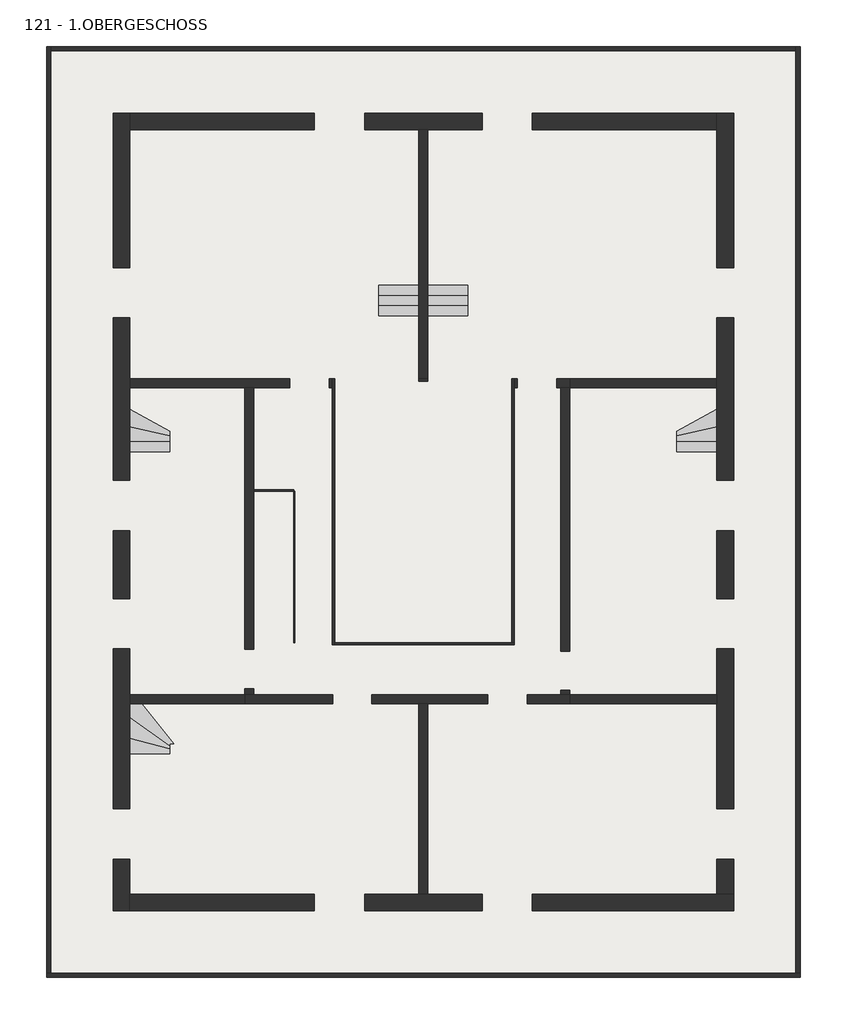
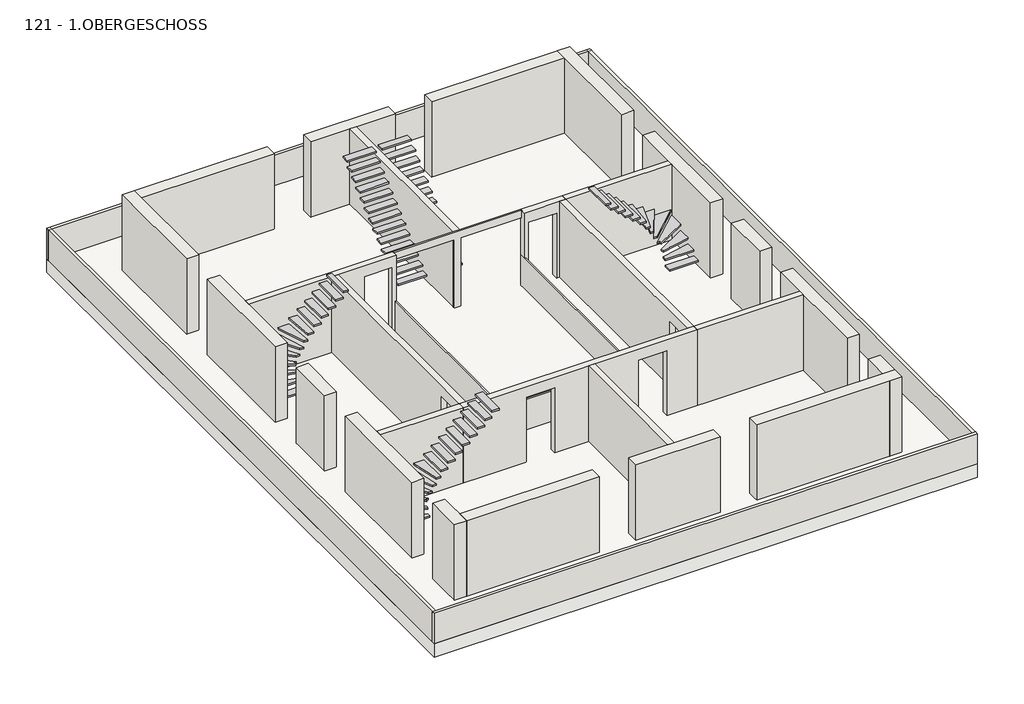
# One storey: 24 walls, 10 stairs, 1 slab.
# Revit data of these elements (continued)
# Type " :1164" (continued)
#   Layers, outside or top first: 0.380 m "holzschalung" (function 1)
# Type " :1165"
#   Layers, outside or top first: 0.380 m "holzschalung" (function 1)
# Type " :1166"
#   Layers, outside or top first: 0.050 m "glas" (function 1)
# Type "Holzwand:1150"
#   ThermalTransmittance = 0.0000 BTU/(h·ft²·°F)
#   Combustible = no
#   Compartmentation = no
#   Layers, outside or top first: 0.200 m "holzschalung" (function 1)
# Type "Holzwand:1151"
#   ThermalTransmittance = 0.0000 BTU/(h·ft²·°F)
#   Combustible = no
#   Compartmentation = no
#   Layers, outside or top first: 0.200 m "holzschalung" (function 1)
# Type "Holzwand:1153"
#   ThermalTransmittance = 0.0000 BTU/(h·ft²·°F)
#   Combustible = no
#   Compartmentation = no
#   Layers, outside or top first: 0.200 m "holzschalung" (function 1)
# Type "Holzwand:1154"
#   ThermalTransmittance = 0.0000 BTU/(h·ft²·°F)
#   Combustible = no
#   Compartmentation = no
#   Layers, outside or top first: 0.030 m "holzschalung" (function 1)
# Type "Holzwand:1155"
#   ThermalTransmittance = 0.0000 BTU/(h·ft²·°F)
#   Combustible = no
#   Compartmentation = no
#   Layers, outside or top first: 0.030 m "holzschalung" (function 1)
# Type "Holzwand:1156"
#   ThermalTransmittance = 0.0000 BTU/(h·ft²·°F)
#   Combustible = no
#   Compartmentation = no
#   Layers, outside or top first: 0.200 m "holzschalung" (function 1)
# Type "Holzwand:1157"
#   ThermalTransmittance = 0.0000 BTU/(h·ft²·°F)
#   Combustible = no
#   Compartmentation = no
#   Layers, outside or top first: 0.200 m "holzschalung" (function 1)
# Type "Holzwand:1158"
#   ThermalTransmittance = 0.0000 BTU/(h·ft²·°F)
#   Combustible = no
#   Compartmentation = no
#   Layers, outside or top first: 0.200 m "holzschalung" (function 1)
# Type "Holzwand:1159"
#   ThermalTransmittance = 0.0000 BTU/(h·ft²·°F)
#   Combustible = no
#   Compartmentation = no
#   Layers, outside or top first: 0.200 m "holzschalung" (function 1)
# Type "Holzwand:1160"
#   ThermalTransmittance = 0.0000 BTU/(h·ft²·°F)
#   Combustible = no
#   Compartmentation = no
#   Layers, outside or top first: 0.200 m "holzschalung" (function 1)
# Type "Holzwand:1162"
#   ThermalTransmittance = 0.0000 BTU/(h·ft²·°F)
#   Combustible = no
#   Compartmentation = no
#   Layers, outside or top first: 0.200 m "holzschalung" (function 1)
# Type "Holzwand:1163"
#   ThermalTransmittance = 0.0000 BTU/(h·ft²·°F)
#   Combustible = no
#   Compartmentation = no
#   Layers, outside or top first: 0.200 m "holzschalung" (function 1)
# Type " :1167"
#   Layers, outside or top first: 0.050 m "holzschalung" (function 1)
# Type " :1168"
#   Layers, outside or top first: 0.050 m "holzschalung" (function 1)
# Type " :1169"
#   Layers, outside or top first: 0.050 m "holzschalung" (function 1)
# Type "Holzwand:1170"
#   ThermalTransmittance = 0.0000 BTU/(h·ft²·°F)
#   Combustible = no
#   Compartmentation = no
#   Layers, outside or top first: 0.100 m "pv - panel anthrazit" (function 1)
# Type "Holzwand:1171"
#   ThermalTransmittance = 0.0000 BTU/(h·ft²·°F)
#   Combustible = no
#   Compartmentation = no
#   Layers, outside or top first: 0.100 m "pv - panel anthrazit" (function 1)
# Type "Holzwand:1172"
#   ThermalTransmittance = 0.0000 BTU/(h·ft²·°F)
#   Combustible = no
#   Compartmentation = no
#   Layers, outside or top first: 0.100 m "pv - panel anthrazit" (function 1)
# Type "Holzwand:1173"
#   ThermalTransmittance = 0.0000 BTU/(h·ft²·°F)
#   Combustible = no
#   Compartmentation = no
#   Layers, outside or top first: 0.100 m "pv - panel anthrazit" (function 1)
# Element 1 (IfcSlab, "Holzdecke 176 : Holzdecke 176")
#   IFC Predefined Type = "FLOOR"
#   Export to IFC As = "ifcslab"
#   IfcGUID = "1_9Us2eVX4OuIZjhNyqdxW"
#   Phase Created = New Construction
#   Materials on its faces: "holzschalung"
# Element 2 (IfcStair, "  97010 :   97010")
#   IFC Predefined Type = "NOTDEFINED"
#   Export to IFC As = "ifcstair"
#   IfcGUID = "2ccaodaeb6QgHPV1d4NBnA"
#   Phase Created = New Construction
#   Materials on its faces: "weiss"
# Element 3 (IfcStair, "  97882 :   97882")
#   IFC Predefined Type = "STRAIGHT_RUN_STAIR"
#   Export to IFC As = "ifcstair"
#   IfcGUID = "1nghyUHoH9yBc_lxkBTUjw"
#   Phase Created = New Construction
#   Materials on its faces: "weiss"
# Element 4 (IfcStair, "  98300 :   98300")
#   IFC Predefined Type = "STRAIGHT_RUN_STAIR"
#   Export to IFC As = "ifcstair"
#   IfcGUID = "2AC_Gmfhz1LvYwUyPOxWan"
#   Phase Created = New Construction
#   Materials on its faces: "weiss"
# Element 5 (IfcStair, "  98728 :   98728")
#   IFC Predefined Type = "NOTDEFINED"
#   Export to IFC As = "ifcstair"
#   IfcGUID = "04Edcgbk9CPwWYiYhycXFf"
#   Phase Created = New Construction
#   Materials on its faces: "weiss"
# Element 6 (IfcStair, "  99154 :   99154")
#   IFC Predefined Type = "NOTDEFINED"
#   Export to IFC As = "ifcstair"
#   IfcGUID = "1azVXxNdn2POY9VYN93ccY"
#   Phase Created = New Construction
#   Materials on its faces: "weiss"
# Element 7 (IfcStair, "  149542 :   149542")
#   IFC Predefined Type = "NOTDEFINED"
#   Export to IFC As = "ifcstair"
#   IfcGUID = "1sH4rJKnLAFOtHPnXrLkif"
#   Phase Created = New Construction
#   Materials on its faces: "weiss"
# Element 8 (IfcStair, "  150414 :   150414")
#   IFC Predefined Type = "STRAIGHT_RUN_STAIR"
#   Export to IFC As = "ifcstair"
#   IfcGUID = "3fdccs_Mj1YAyFFpBc3gyk"
#   Phase Created = New Construction
#   Materials on its faces: "weiss"
# Element 9 (IfcStair, "  150832 :   150832")
#   IFC Predefined Type = "STRAIGHT_RUN_STAIR"
#   Export to IFC As = "ifcstair"
#   IfcGUID = "2szmEZdbD3KBDvfX1Sa6Vh"
#   Phase Created = New Construction
#   Materials on its faces: "weiss"
# Element 10 (IfcStair, "  151260 :   151260")
#   IFC Predefined Type = "NOTDEFINED"
#   Export to IFC As = "ifcstair"
#   IfcGUID = "1YKyaFTbr8YR41yGjubBsl"
#   Phase Created = New Construction
#   Materials on its faces: "weiss"
# Element 11 (IfcStair, "  151686 :   151686")
#   IFC Predefined Type = "NOTDEFINED"
#   Export to IFC As = "ifcstair"
#   IfcGUID = "2KPGRYHzzCygzBebAeLtPz"
#   Phase Created = New Construction
#   Materials on its faces: "weiss"
# Element 12 (IfcWall, " :1152")
#   Export to IFC As = "ifcwall"
#   IfcGUID = "2CeDj8YZTCPx$yj4WDVOez"
#   NameOverride = " "
#   Abrechnungsart = "m³"
#   Allright_Bauteil_ID = "0121HWa0785064286"
#   Layer #1:Object Layer Attributes #1:Abrechnungsart = "m²"
#   Layer #1:Object Layer Attributes #1:Allright_Bauteil_ID = "0121Wa 0785064367"
#   Layer #1:Object Layer Attributes #1:Gewerk = "Zimmer- und Holzbauarbeiten"
#   Layer #1:Object Layer Attributes #1:Material = "k.Ausw."
#   Layer #1:Object Layer Attributes #1:Objektname = "Wand"
#   Layer #1:Object Layer Attributes #1:Status = "Neubau"
#   MEP Wandtyp = "HO-WA-HSW\\"
#   Objektname = "Gesamtwand"
#   built-in parameter 1001111 = 0.505 m
#   Top Offset = 0.000 m
#   Base Offset = 0.505 m
#   Unconnected Height = 2.500 m
#   wall height = 2.500 m
#   Layer #1:Object Layer Attributes #1:2D Interaktion = yes
#   Phase Created = New Construction
#   Base Constraint = 121 - 1.OBERGESCHOSS
#   Materials on its faces: "holzschalung"
# Element 13 (IfcWall, " :1161")
#   Export to IFC As = "ifcwall"
#   IfcGUID = "2TnImcbz91shb3jN7Wgb8B"
#   NameOverride = " "
#   Abrechnungsart = "m³"
#   Allright_Bauteil_ID = "0121HWa0785064349"
#   Layer #1:Object Layer Attributes #1:Abrechnungsart = "m²"
#   Layer #1:Object Layer Attributes #1:Allright_Bauteil_ID = "0121Wa 0785064397"
#   Layer #1:Object Layer Attributes #1:Gewerk = "Zimmer- und Holzbauarbeiten"
#   Layer #1:Object Layer Attributes #1:Material = "k.Ausw."
#   Layer #1:Object Layer Attributes #1:Objektname = "Wand"
#   Layer #1:Object Layer Attributes #1:Status = "Neubau"
#   MEP Wandtyp = "HO-WA-HSW\\"
#   Objektname = "Gesamtwand"
#   built-in parameter 1001111 = 0.505 m
#   Top Offset = 0.000 m
#   Base Offset = 0.505 m
#   Unconnected Height = 2.500 m
#   wall height = 2.500 m
#   Layer #1:Object Layer Attributes #1:2D Interaktion = yes
#   Phase Created = New Construction
#   Base Constraint = 121 - 1.OBERGESCHOSS
#   Materials on its faces: "holzschalung"
# Element 14 (IfcWall, " :1164")
#   Export to IFC As = "ifcwall"
#   IfcGUID = "1tWRh4hxLAdASVw4VNE3to"
#   NameOverride = " "
#   Abrechnungsart = "m³"
#   Allright_Bauteil_ID = "0121HWa0785092952"
#   Layer #1:Object Layer Attributes #1:Abrechnungsart = "m²"
#   Layer #1:Object Layer Attributes #1:Allright_Bauteil_ID = "0121Wa 0785092986"
#   Layer #1:Object Layer Attributes #1:Gewerk = "Zimmer- und Holzbauarbeiten"
#   Layer #1:Object Layer Attributes #1:Material = "k.Ausw."
#   Layer #1:Object Layer Attributes #1:Objektname = "Wand"
#   Layer #1:Object Layer Attributes #1:Status = "Neubau"
#   MEP Wandtyp = "HO-WA-HSW\\"
#   Objektname = "Gesamtwand"
#   built-in parameter 1001111 = 0.505 m
#   Top Offset = 0.000 m
#   Base Offset = 0.505 m
#   Unconnected Height = 2.500 m
#   wall height = 2.500 m
#   Layer #1:Object Layer Attributes #1:2D Interaktion = yes
#   Phase Created = New Construction
#   Base Constraint = 121 - 1.OBERGESCHOSS
#   Materials on its faces: "holzschalung"
# Element 15 (IfcWall, " :1165")
#   Export to IFC As = "ifcwall"
#   IfcGUID = "1HE73MTmDEEBf4AV7ughZ8"
#   NameOverride = " "
#   Abrechnungsart = "m³"
#   Allright_Bauteil_ID = "0121HWa0785097898"
#   Layer #1:Object Layer Attributes #1:Abrechnungsart = "m²"
#   Layer #1:Object Layer Attributes #1:Allright_Bauteil_ID = "0121Wa 0785097934"
#   Layer #1:Object Layer Attributes #1:Gewerk = "Zimmer- und Holzbauarbeiten"
#   Layer #1:Object Layer Attributes #1:Material = "k.Ausw."
#   Layer #1:Object Layer Attributes #1:Objektname = "Wand"
#   Layer #1:Object Layer Attributes #1:Status = "Neubau"
#   MEP Wandtyp = "HO-WA-HSW\\"
#   Objektname = "Gesamtwand"
#   built-in parameter 1001111 = 0.505 m
#   Top Offset = 0.000 m
#   Base Offset = 0.505 m
#   Unconnected Height = 2.500 m
#   wall height = 2.500 m
#   Layer #1:Object Layer Attributes #1:2D Interaktion = yes
#   Phase Created = New Construction
#   Base Constraint = 121 - 1.OBERGESCHOSS
#   Materials on its faces: "holzschalung"
# Element 16 (IfcWall, " :1166")
#   Export to IFC As = "ifcwall"
#   IfcGUID = "0t2qqx1kvDZPNPdKl4bfzP"
#   NameOverride = " "
#   Abrechnungsart = "m³"
#   Allright_Bauteil_ID = "0121HWa0785064296"
#   Layer #1:Object Layer Attributes #1:Abrechnungsart = "m²"
#   Layer #1:Object Layer Attributes #1:Allright_Bauteil_ID = "0121Wa 0785064386"
#   Layer #1:Object Layer Attributes #1:Gewerk = "Zimmer- und Holzbauarbeiten"
#   Layer #1:Object Layer Attributes #1:Material = "k.Ausw."
#   Layer #1:Object Layer Attributes #1:Objektname = "Wand"
#   Layer #1:Object Layer Attributes #1:Status = "Neubau"
#   MEP Wandtyp = "HO-WA-HSW\\"
#   Objektname = "Gesamtwand"
#   built-in parameter 1001111 = 0.505 m
#   Top Offset = 0.000 m
#   Base Offset = 0.505 m
#   Unconnected Height = 2.500 m
#   wall height = 2.500 m
#   Layer #1:Object Layer Attributes #1:2D Interaktion = yes
#   Phase Created = New Construction
#   Base Constraint = 121 - 1.OBERGESCHOSS
#   Materials on its faces: "glas"
# Element 17 (IfcWall, "Holzwand:1150")
#   Export to IFC As = "ifcwall"
#   IfcGUID = "3nZ5Mon9nBjwoRgvyoor9a"
#   NameOverride = "Holzwand"
#   Abrechnungsart = "St"
#   Allright_Bauteil_ID = "0121HWa0785065367"
#   Bezeichnung = "Holzwand"
#   Layer #1:Object Layer Attributes #1:Abrechnungsart = "m²"
#   Layer #1:Object Layer Attributes #1:Allright_Bauteil_ID = "0121Wa 0785065369"
#   Layer #1:Object Layer Attributes #1:Bezeichnung = "Holzwand"
#   Layer #1:Object Layer Attributes #1:Codetext = "HO-WI-HSW\\"
#   Layer #1:Object Layer Attributes #1:Gewerk = "Zimmer- und Holzbauarbeiten"
#   Layer #1:Object Layer Attributes #1:Material = "Holz"
#   Layer #1:Object Layer Attributes #1:Objektname = "Wand"
#   Layer #1:Object Layer Attributes #1:Reference = "Holzwand"
#   Layer #1:Object Layer Attributes #1:Status = "Neubau"
#   MEP Wandtyp = "HO-WA-HSW\\"
#   Objektname = "Gesamtwand"
#   Reference = "Holzwand"
#   Status = "NEW"
#   built-in parameter 1001111 = 0.505 m
#   Top Offset = 0.000 m
#   Base Offset = 0.505 m
#   Unconnected Height = 2.500 m
#   wall height = 2.500 m
#   Layer #1:Object Layer Attributes #1:U-Wert = 0
#   Layer #1:Object Layer Attributes #1:2D Interaktion = yes
#   Layer #1:Object Layer Attributes #1:Außenbauteil = no
#   Layer #1:Object Layer Attributes #1:Brandabschnittsdefinierendes Bauteil = no
#   Layer #1:Object Layer Attributes #1:Brennbares Material = no
#   Layer #1:Object Layer Attributes #1:Raumhohe Wand = yes
#   Layer #1:Object Layer Attributes #1:Tragendes Bauteil = yes
#   ExtendToStructure = yes
#   IsExternal = no
#   LoadBearing = yes
#   Phase Created = New Construction
#   Base Constraint = 121 - 1.OBERGESCHOSS
#   Materials on its faces: "holzschalung"
# Element 18 (IfcWall, "Holzwand:1151")
#   Export to IFC As = "ifcwall"
#   IfcGUID = "3jE1E$NFj7vAP$vn70kdrt"
#   NameOverride = "Holzwand"
#   Abrechnungsart = "St"
#   Allright_Bauteil_ID = "0121HWa0785066899"
#   Bezeichnung = "Holzwand"
#   Layer #1:Object Layer Attributes #1:Abrechnungsart = "m²"
#   Layer #1:Object Layer Attributes #1:Allright_Bauteil_ID = "0121Wa 0785066901"
#   Layer #1:Object Layer Attributes #1:Bezeichnung = "Holzwand"
#   Layer #1:Object Layer Attributes #1:Codetext = "HO-WI-HSW\\"
#   Layer #1:Object Layer Attributes #1:Gewerk = "Zimmer- und Holzbauarbeiten"
#   Layer #1:Object Layer Attributes #1:Material = "Holz"
#   Layer #1:Object Layer Attributes #1:Objektname = "Wand"
#   Layer #1:Object Layer Attributes #1:Reference = "Holzwand"
#   Layer #1:Object Layer Attributes #1:Status = "Neubau"
#   MEP Wandtyp = "HO-WA-HSW\\"
#   Objektname = "Gesamtwand"
#   Reference = "Holzwand"
#   Status = "NEW"
#   built-in parameter 1001111 = 0.505 m
#   Top Offset = 0.000 m
#   Base Offset = 0.505 m
#   Unconnected Height = 2.500 m
#   wall height = 2.500 m
#   Layer #1:Object Layer Attributes #1:U-Wert = 0
#   Layer #1:Object Layer Attributes #1:2D Interaktion = yes
#   Layer #1:Object Layer Attributes #1:Außenbauteil = no
#   Layer #1:Object Layer Attributes #1:Brandabschnittsdefinierendes Bauteil = no
#   Layer #1:Object Layer Attributes #1:Brennbares Material = no
#   Layer #1:Object Layer Attributes #1:Raumhohe Wand = yes
#   Layer #1:Object Layer Attributes #1:Tragendes Bauteil = yes
#   ExtendToStructure = yes
#   IsExternal = no
#   LoadBearing = yes
#   Phase Created = New Construction
#   Base Constraint = 121 - 1.OBERGESCHOSS
#   Materials on its faces: "holzschalung"
# Element 19 (IfcWall, "Holzwand:1153")
#   Export to IFC As = "ifcwall"
#   IfcGUID = "1Zhxv5EALB9e6_$pCtUEXg"
#   NameOverride = "Holzwand"
#   Abrechnungsart = "St"
#   Allright_Bauteil_ID = "0121HWa0785065540"
#   Bezeichnung = "Holzwand"
#   Layer #1:Object Layer Attributes #1:Abrechnungsart = "m²"
#   Layer #1:Object Layer Attributes #1:Allright_Bauteil_ID = "0121Wa 0785065541"
#   Layer #1:Object Layer Attributes #1:Bezeichnung = "Holzwand"
#   Layer #1:Object Layer Attributes #1:Codetext = "HO-WI-HSW\\"
#   Layer #1:Object Layer Attributes #1:Gewerk = "Zimmer- und Holzbauarbeiten"
#   Layer #1:Object Layer Attributes #1:Material = "Holz"
#   Layer #1:Object Layer Attributes #1:Objektname = "Wand"
#   Layer #1:Object Layer Attributes #1:Reference = "Holzwand"
#   Layer #1:Object Layer Attributes #1:Status = "Neubau"
#   MEP Wandtyp = "HO-WA-HSW\\"
#   Objektname = "Gesamtwand"
#   Reference = "Holzwand"
#   Status = "NEW"
#   built-in parameter 1001111 = 0.505 m
#   Top Offset = 0.000 m
#   Base Offset = 0.505 m
#   Unconnected Height = 2.500 m
#   wall height = 2.500 m
#   Layer #1:Object Layer Attributes #1:U-Wert = 0
#   Layer #1:Object Layer Attributes #1:2D Interaktion = yes
#   Layer #1:Object Layer Attributes #1:Außenbauteil = no
#   Layer #1:Object Layer Attributes #1:Brandabschnittsdefinierendes Bauteil = no
#   Layer #1:Object Layer Attributes #1:Brennbares Material = no
#   Layer #1:Object Layer Attributes #1:Raumhohe Wand = yes
#   Layer #1:Object Layer Attributes #1:Tragendes Bauteil = yes
#   ExtendToStructure = yes
#   IsExternal = no
#   LoadBearing = yes
#   Phase Created = New Construction
#   Base Constraint = 121 - 1.OBERGESCHOSS
#   Materials on its faces: "holzschalung"
# Element 20 (IfcWall, "Holzwand:1154")
#   Export to IFC As = "ifcwall"
#   IfcGUID = "2MsVq3EJn0K8wHdQ6uoxnd"
#   NameOverride = "Holzwand"
#   Abrechnungsart = "St"
#   Allright_Bauteil_ID = "0121HWa0785067355"
#   Bezeichnung = "Holzwand"
#   Layer #1:Object Layer Attributes #1:Abrechnungsart = "m²"
#   Layer #1:Object Layer Attributes #1:Allright_Bauteil_ID = "0121Wa 0785067356"
#   Layer #1:Object Layer Attributes #1:Codetext = "HO-WI-HSW\\"
#   Layer #1:Object Layer Attributes #1:Gewerk = "Zimmer- und Holzbauarbeiten"
#   Layer #1:Object Layer Attributes #1:Material = "Holz"
#   Layer #1:Object Layer Attributes #1:Objektname = "Wand"
#   Layer #1:Object Layer Attributes #1:Reference = "Holzwand"
#   Layer #1:Object Layer Attributes #1:Status = "Neubau"
#   MEP Wandtyp = "HO-WA-HSW\\"
#   Objektname = "Gesamtwand"
#   Reference = "Holzwand"
#   Status = "NEW"
#   built-in parameter 1001111 = 0.505 m
#   Top Offset = 0.000 m
#   Base Offset = 0.505 m
#   Unconnected Height = 1.000 m
#   wall height = 1.000 m
#   Layer #1:Object Layer Attributes #1:U-Wert = 0
#   Layer #1:Object Layer Attributes #1:2D Interaktion = yes
#   Layer #1:Object Layer Attributes #1:Außenbauteil = no
#   Layer #1:Object Layer Attributes #1:Brandabschnittsdefinierendes Bauteil = no
#   Layer #1:Object Layer Attributes #1:Brennbares Material = no
#   Layer #1:Object Layer Attributes #1:Raumhohe Wand = yes
#   ExtendToStructure = yes
#   IsExternal = no
#   LoadBearing = yes
#   Phase Created = New Construction
#   Base Constraint = 121 - 1.OBERGESCHOSS
#   Materials on its faces: "holzschalung"
# Element 21 (IfcWall, "Holzwand:1155")
#   Export to IFC As = "ifcwall"
#   IfcGUID = "1F_ySrDsP9oP3MqXymSTVO"
#   NameOverride = "Holzwand"
#   Abrechnungsart = "St"
#   Allright_Bauteil_ID = "0121HWa0785067347"
#   Bezeichnung = "Holzwand"
#   Layer #1:Object Layer Attributes #1:Abrechnungsart = "m²"
#   Layer #1:Object Layer Attributes #1:Allright_Bauteil_ID = "0121Wa 0785067348"
#   Layer #1:Object Layer Attributes #1:Codetext = "HO-WI-HSW\\"
#   Layer #1:Object Layer Attributes #1:Gewerk = "Zimmer- und Holzbauarbeiten"
#   Layer #1:Object Layer Attributes #1:Material = "Holz"
#   Layer #1:Object Layer Attributes #1:Objektname = "Wand"
#   Layer #1:Object Layer Attributes #1:Reference = "Holzwand"
#   Layer #1:Object Layer Attributes #1:Status = "Neubau"
#   MEP Wandtyp = "HO-WA-HSW\\"
#   Objektname = "Gesamtwand"
#   Reference = "Holzwand"
#   Status = "NEW"
#   built-in parameter 1001111 = 0.505 m
#   Top Offset = 0.000 m
#   Base Offset = 0.505 m
#   Unconnected Height = 1.000 m
#   wall height = 1.000 m
#   Layer #1:Object Layer Attributes #1:U-Wert = 0
#   Layer #1:Object Layer Attributes #1:2D Interaktion = yes
#   Layer #1:Object Layer Attributes #1:Außenbauteil = no
#   Layer #1:Object Layer Attributes #1:Brandabschnittsdefinierendes Bauteil = no
#   Layer #1:Object Layer Attributes #1:Brennbares Material = no
#   Layer #1:Object Layer Attributes #1:Raumhohe Wand = yes
#   ExtendToStructure = yes
#   IsExternal = no
#   LoadBearing = yes
#   Phase Created = New Construction
#   Base Constraint = 121 - 1.OBERGESCHOSS
#   Materials on its faces: "holzschalung"
# Element 22 (IfcWall, "Holzwand:1156")
#   Export to IFC As = "ifcwall"
#   IfcGUID = "0gtwZwppj1pObqyI7HY41_"
#   NameOverride = "Holzwand"
#   Abrechnungsart = "St"
#   Allright_Bauteil_ID = "0121HWa0785064323"
#   Bezeichnung = "Holzwand"
#   Layer #1:Object Layer Attributes #1:Abrechnungsart = "m²"
#   Layer #1:Object Layer Attributes #1:Allright_Bauteil_ID = "0121Wa 0785064369"
#   Layer #1:Object Layer Attributes #1:Bezeichnung = "Holzwand"
#   Layer #1:Object Layer Attributes #1:Codetext = "HO-WI-HSW\\"
#   Layer #1:Object Layer Attributes #1:Gewerk = "Zimmer- und Holzbauarbeiten"
#   Layer #1:Object Layer Attributes #1:Material = "Holz"
#   Layer #1:Object Layer Attributes #1:Objektname = "Wand"
#   Layer #1:Object Layer Attributes #1:Reference = "Holzwand"
#   Layer #1:Object Layer Attributes #1:Status = "Neubau"
#   MEP Wandtyp = "HO-WA-HSW\\"
#   Objektname = "Gesamtwand"
#   Reference = "Holzwand"
#   Status = "NEW"
#   built-in parameter 1001111 = 0.505 m
#   Top Offset = 0.000 m
#   Base Offset = 0.505 m
#   Unconnected Height = 2.500 m
#   wall height = 2.500 m
#   Layer #1:Object Layer Attributes #1:U-Wert = 0
#   Layer #1:Object Layer Attributes #1:2D Interaktion = yes
#   Layer #1:Object Layer Attributes #1:Außenbauteil = no
#   Layer #1:Object Layer Attributes #1:Brandabschnittsdefinierendes Bauteil = no
#   Layer #1:Object Layer Attributes #1:Brennbares Material = no
#   Layer #1:Object Layer Attributes #1:Raumhohe Wand = yes
#   Layer #1:Object Layer Attributes #1:Tragendes Bauteil = yes
#   ExtendToStructure = yes
#   IsExternal = no
#   LoadBearing = yes
#   Phase Created = New Construction
#   Base Constraint = 121 - 1.OBERGESCHOSS
#   Materials on its faces: "holzschalung"
# Element 23 (IfcWall, "Holzwand:1157")
#   Export to IFC As = "ifcwall"
#   IfcGUID = "0tY6$O1l121AktLhYSWZjf"
#   NameOverride = "Holzwand"
#   Abrechnungsart = "St"
#   Allright_Bauteil_ID = "0121HWa0785064381"
#   Bezeichnung = "Holzwand"
#   Layer #1:Object Layer Attributes #1:Abrechnungsart = "m²"
#   Layer #1:Object Layer Attributes #1:Allright_Bauteil_ID = "0121Wa 0785064384"
#   Layer #1:Object Layer Attributes #1:Bezeichnung = "Holzwand"
#   Layer #1:Object Layer Attributes #1:Codetext = "HO-WI-HSW\\"
#   Layer #1:Object Layer Attributes #1:Gewerk = "Zimmer- und Holzbauarbeiten"
#   Layer #1:Object Layer Attributes #1:Material = "Holz"
#   Layer #1:Object Layer Attributes #1:Objektname = "Wand"
#   Layer #1:Object Layer Attributes #1:Reference = "Holzwand"
#   Layer #1:Object Layer Attributes #1:Status = "Neubau"
#   MEP Wandtyp = "HO-WA-HSW\\"
#   Objektname = "Gesamtwand"
#   Reference = "Holzwand"
#   Status = "NEW"
#   built-in parameter 1001111 = 0.505 m
#   Top Offset = 0.000 m
#   Base Offset = 0.505 m
#   Unconnected Height = 2.500 m
#   wall height = 2.500 m
#   Layer #1:Object Layer Attributes #1:U-Wert = 0
#   Layer #1:Object Layer Attributes #1:2D Interaktion = yes
#   Layer #1:Object Layer Attributes #1:Außenbauteil = no
#   Layer #1:Object Layer Attributes #1:Brandabschnittsdefinierendes Bauteil = no
#   Layer #1:Object Layer Attributes #1:Brennbares Material = no
#   Layer #1:Object Layer Attributes #1:Raumhohe Wand = yes
#   Layer #1:Object Layer Attributes #1:Tragendes Bauteil = yes
#   ExtendToStructure = yes
#   IsExternal = no
#   LoadBearing = yes
#   Phase Created = New Construction
#   Base Constraint = 121 - 1.OBERGESCHOSS
#   Materials on its faces: "holzschalung"
# Element 24 (IfcWall, "Holzwand:1158")
#   Export to IFC As = "ifcwall"
#   IfcGUID = "2Mr8L52dj4iP8MoJTiOa9p"
#   NameOverride = "Holzwand"
#   Abrechnungsart = "St"
#   Allright_Bauteil_ID = "0121HWa0785069286"
#   Bezeichnung = "Holzwand"
#   Layer #1:Object Layer Attributes #1:Abrechnungsart = "m²"
#   Layer #1:Object Layer Attributes #1:Allright_Bauteil_ID = "0121Wa 0785069294"
#   Layer #1:Object Layer Attributes #1:Bezeichnung = "Holzwand"
#   Layer #1:Object Layer Attributes #1:Codetext = "HO-WI-HSW\\"
#   Layer #1:Object Layer Attributes #1:Gewerk = "Zimmer- und Holzbauarbeiten"
#   Layer #1:Object Layer Attributes #1:Material = "Holz"
#   Layer #1:Object Layer Attributes #1:Objektname = "Wand"
#   Layer #1:Object Layer Attributes #1:Reference = "Holzwand"
#   Layer #1:Object Layer Attributes #1:Status = "Neubau"
#   MEP Wandtyp = "HO-WA-HSW\\"
#   Objektname = "Gesamtwand"
#   Reference = "Holzwand"
#   Status = "NEW"
#   built-in parameter 1001111 = 0.505 m
#   Top Offset = 0.000 m
#   Base Offset = 0.505 m
#   Unconnected Height = 2.500 m
#   wall height = 2.500 m
#   Layer #1:Object Layer Attributes #1:U-Wert = 0
#   Layer #1:Object Layer Attributes #1:2D Interaktion = yes
#   Layer #1:Object Layer Attributes #1:Außenbauteil = no
#   Layer #1:Object Layer Attributes #1:Brandabschnittsdefinierendes Bauteil = no
#   Layer #1:Object Layer Attributes #1:Brennbares Material = no
#   Layer #1:Object Layer Attributes #1:Raumhohe Wand = yes
#   Layer #1:Object Layer Attributes #1:Tragendes Bauteil = yes
#   ExtendToStructure = yes
#   IsExternal = no
#   LoadBearing = yes
#   Phase Created = New Construction
#   Base Constraint = 121 - 1.OBERGESCHOSS
#   Materials on its faces: "holzschalung"
# Element 25 (IfcWall, "Holzwand:1159")
#   Export to IFC As = "ifcwall"
#   IfcGUID = "36leNf4gL9OB_v358ffY76"
#   NameOverride = "Holzwand"
#   Abrechnungsart = "St"
#   Allright_Bauteil_ID = "0121HWa0785064324"
#   Bezeichnung = "Holzwand"
#   Layer #1:Object Layer Attributes #1:Abrechnungsart = "m²"
#   Layer #1:Object Layer Attributes #1:Allright_Bauteil_ID = "0121Wa 0785064395"
#   Layer #1:Object Layer Attributes #1:Bezeichnung = "Holzwand"
#   Layer #1:Object Layer Attributes #1:Codetext = "HO-WI-HSW\\"
#   Layer #1:Object Layer Attributes #1:Gewerk = "Zimmer- und Holzbauarbeiten"
#   Layer #1:Object Layer Attributes #1:Material = "Holz"
#   Layer #1:Object Layer Attributes #1:Objektname = "Wand"
#   Layer #1:Object Layer Attributes #1:Reference = "Holzwand"
#   Layer #1:Object Layer Attributes #1:Status = "Neubau"
#   MEP Wandtyp = "HO-WA-HSW\\"
#   Objektname = "Gesamtwand"
#   Reference = "Holzwand"
#   Status = "NEW"
#   built-in parameter 1001111 = 0.505 m
#   Top Offset = 0.000 m
#   Base Offset = 0.505 m
#   Unconnected Height = 2.500 m
#   wall height = 2.500 m
#   Layer #1:Object Layer Attributes #1:U-Wert = 0
#   Layer #1:Object Layer Attributes #1:2D Interaktion = yes
#   Layer #1:Object Layer Attributes #1:Außenbauteil = no
#   Layer #1:Object Layer Attributes #1:Brandabschnittsdefinierendes Bauteil = no
#   Layer #1:Object Layer Attributes #1:Brennbares Material = no
#   Layer #1:Object Layer Attributes #1:Raumhohe Wand = yes
#   Layer #1:Object Layer Attributes #1:Tragendes Bauteil = yes
#   ExtendToStructure = yes
#   IsExternal = no
#   LoadBearing = yes
#   Phase Created = New Construction
#   Base Constraint = 121 - 1.OBERGESCHOSS
#   Materials on its faces: "holzschalung"
# Element 26 (IfcWall, "Holzwand:1160")
#   Export to IFC As = "ifcwall"
#   IfcGUID = "3kHHpx_NTE_9JnfL3dFkYB"
#   NameOverride = "Holzwand"
#   Abrechnungsart = "St"
#   Allright_Bauteil_ID = "0121HWa0785064389"
#   Bezeichnung = "Holzwand"
#   Layer #1:Object Layer Attributes #1:Abrechnungsart = "m²"
#   Layer #1:Object Layer Attributes #1:Allright_Bauteil_ID = "0121Wa 0785064393"
#   Layer #1:Object Layer Attributes #1:Bezeichnung = "Holzwand"
#   Layer #1:Object Layer Attributes #1:Codetext = "HO-WI-HSW\\"
#   Layer #1:Object Layer Attributes #1:Gewerk = "Zimmer- und Holzbauarbeiten"
#   Layer #1:Object Layer Attributes #1:Material = "Holz"
#   Layer #1:Object Layer Attributes #1:Objektname = "Wand"
#   Layer #1:Object Layer Attributes #1:Reference = "Holzwand"
#   Layer #1:Object Layer Attributes #1:Status = "Neubau"
#   MEP Wandtyp = "HO-WA-HSW\\"
#   Objektname = "Gesamtwand"
#   Reference = "Holzwand"
#   Status = "NEW"
#   built-in parameter 1001111 = 0.505 m
#   Top Offset = 0.000 m
#   Base Offset = 0.505 m
#   Unconnected Height = 2.500 m
#   wall height = 2.500 m
#   Layer #1:Object Layer Attributes #1:U-Wert = 0
#   Layer #1:Object Layer Attributes #1:2D Interaktion = yes
#   Layer #1:Object Layer Attributes #1:Außenbauteil = no
#   Layer #1:Object Layer Attributes #1:Brandabschnittsdefinierendes Bauteil = no
#   Layer #1:Object Layer Attributes #1:Brennbares Material = no
#   Layer #1:Object Layer Attributes #1:Raumhohe Wand = yes
#   Layer #1:Object Layer Attributes #1:Tragendes Bauteil = yes
#   ExtendToStructure = yes
#   IsExternal = no
#   LoadBearing = yes
#   Phase Created = New Construction
#   Base Constraint = 121 - 1.OBERGESCHOSS
#   Materials on its faces: "holzschalung"
# Element 27 (IfcWall, "Holzwand:1162")
#   Export to IFC As = "ifcwall"
#   IfcGUID = "26lQuimMP00PZvPhbBRI2R"
#   NameOverride = "Holzwand"
#   Abrechnungsart = "St"
#   Allright_Bauteil_ID = "0121HWa0785065329"
#   Bezeichnung = "Holzwand"
#   Layer #1:Object Layer Attributes #1:Abrechnungsart = "m²"
#   Layer #1:Object Layer Attributes #1:Allright_Bauteil_ID = "0121Wa 0785065331"
#   Layer #1:Object Layer Attributes #1:Bezeichnung = "Holzwand"
#   Layer #1:Object Layer Attributes #1:Codetext = "HO-WI-HSW\\"
#   Layer #1:Object Layer Attributes #1:Gewerk = "Zimmer- und Holzbauarbeiten"
#   Layer #1:Object Layer Attributes #1:Material = "Holz"
#   Layer #1:Object Layer Attributes #1:Objektname = "Wand"
#   Layer #1:Object Layer Attributes #1:Reference = "Holzwand"
#   Layer #1:Object Layer Attributes #1:Status = "Neubau"
#   MEP Wandtyp = "HO-WA-HSW\\"
#   Objektname = "Gesamtwand"
#   Reference = "Holzwand"
#   Status = "NEW"
#   built-in parameter 1001111 = 0.505 m
#   Top Offset = 0.000 m
#   Base Offset = 0.505 m
#   Unconnected Height = 2.500 m
#   wall height = 2.500 m
#   Layer #1:Object Layer Attributes #1:U-Wert = 0
#   Layer #1:Object Layer Attributes #1:2D Interaktion = yes
#   Layer #1:Object Layer Attributes #1:Außenbauteil = no
#   Layer #1:Object Layer Attributes #1:Brandabschnittsdefinierendes Bauteil = no
#   Layer #1:Object Layer Attributes #1:Brennbares Material = no
#   Layer #1:Object Layer Attributes #1:Raumhohe Wand = yes
#   Layer #1:Object Layer Attributes #1:Tragendes Bauteil = yes
#   ExtendToStructure = yes
#   IsExternal = no
#   LoadBearing = yes
#   Phase Created = New Construction
#   Base Constraint = 121 - 1.OBERGESCHOSS
#   Materials on its faces: "holzschalung"
# Element 28 (IfcWall, "Holzwand:1163")
#   Export to IFC As = "ifcwall"
#   IfcGUID = "3atU$IMTH8YP$GZozT8ehc"
#   NameOverride = "Holzwand"
#   Abrechnungsart = "St"
#   Allright_Bauteil_ID = "0121HWa0785064334"
#   Bezeichnung = "Holzwand"
#   Layer #1:Object Layer Attributes #1:Abrechnungsart = "m²"
#   Layer #1:Object Layer Attributes #1:Allright_Bauteil_ID = "0121Wa 0785064371"
#   Layer #1:Object Layer Attributes #1:Bezeichnung = "Holzwand"
#   Layer #1:Object Layer Attributes #1:Codetext = "HO-WI-HSW\\"
#   Layer #1:Object Layer Attributes #1:Gewerk = "Zimmer- und Holzbauarbeiten"
#   Layer #1:Object Layer Attributes #1:Material = "Holz"
#   Layer #1:Object Layer Attributes #1:Objektname = "Wand"
#   Layer #1:Object Layer Attributes #1:Reference = "Holzwand"
#   Layer #1:Object Layer Attributes #1:Status = "Neubau"
#   MEP Wandtyp = "HO-WA-HSW\\"
#   Objektname = "Gesamtwand"
#   Reference = "Holzwand"
#   Status = "NEW"
#   built-in parameter 1001111 = 0.505 m
#   Top Offset = 0.000 m
#   Base Offset = 0.505 m
#   Unconnected Height = 2.500 m
#   wall height = 2.500 m
#   Layer #1:Object Layer Attributes #1:U-Wert = 0
#   Layer #1:Object Layer Attributes #1:2D Interaktion = yes
#   Layer #1:Object Layer Attributes #1:Außenbauteil = no
#   Layer #1:Object Layer Attributes #1:Brandabschnittsdefinierendes Bauteil = no
#   Layer #1:Object Layer Attributes #1:Brennbares Material = no
#   Layer #1:Object Layer Attributes #1:Raumhohe Wand = yes
#   Layer #1:Object Layer Attributes #1:Tragendes Bauteil = yes
#   ExtendToStructure = yes
#   IsExternal = no
#   LoadBearing = yes
#   Phase Created = New Construction
#   Base Constraint = 121 - 1.OBERGESCHOSS
#   Materials on its faces: "holzschalung"
# Element 29 (IfcWall, " :1167")
#   Export to IFC As = "ifcwall"
#   IfcGUID = "35Iolt9MTFw82QPYPk5JvU"
#   NameOverride = " "
#   Abrechnungsart = "m³"
#   Allright_Bauteil_ID = "0121HWa0785064294"
#   Layer #1:Object Layer Attributes #1:Abrechnungsart = "m²"
#   Layer #1:Object Layer Attributes #1:Allright_Bauteil_ID = "0121Wa 0785064340"
#   Layer #1:Object Layer Attributes #1:Gewerk = "Zimmer- und Holzbauarbeiten"
#   Layer #1:Object Layer Attributes #1:Material = "k.Ausw."
#   Layer #1:Object Layer Attributes #1:Objektname = "Wand"
#   Layer #1:Object Layer Attributes #1:Status = "Neubau"
#   MEP Wandtyp = "HO-WA-HSW\\"
#   Objektname = "Gesamtwand"
#   built-in parameter 1001111 = 0.505 m
#   Top Offset = 0.000 m
#   Base Offset = 0.505 m
#   Unconnected Height = 1.000 m
#   wall height = 1.000 m
#   Layer #1:Object Layer Attributes #1:2D Interaktion = yes
#   Layer #1:Object Layer Attributes #1:Tragendes Bauteil = no
#   Phase Created = New Construction
#   Base Constraint = 121 - 1.OBERGESCHOSS
#   Materials on its faces: "holzschalung"
# Element 30 (IfcWall, " :1168")
#   Export to IFC As = "ifcwall"
#   IfcGUID = "21NDiotIv7sAO2c5Bbio25"
#   NameOverride = " "
#   Abrechnungsart = "m³"
#   Allright_Bauteil_ID = "0121HWa0785064290"
#   Layer #1:Object Layer Attributes #1:Abrechnungsart = "m²"
#   Layer #1:Object Layer Attributes #1:Allright_Bauteil_ID = "0121Wa 0785064348"
#   Layer #1:Object Layer Attributes #1:Gewerk = "Zimmer- und Holzbauarbeiten"
#   Layer #1:Object Layer Attributes #1:Material = "k.Ausw."
#   Layer #1:Object Layer Attributes #1:Objektname = "Wand"
#   Layer #1:Object Layer Attributes #1:Status = "Neubau"
#   MEP Wandtyp = "HO-WA-HSW\\"
#   Objektname = "Gesamtwand"
#   built-in parameter 1001111 = 0.505 m
#   Top Offset = 0.000 m
#   Base Offset = 0.505 m
#   Unconnected Height = 1.000 m
#   wall height = 1.000 m
#   Layer #1:Object Layer Attributes #1:2D Interaktion = yes
#   Layer #1:Object Layer Attributes #1:Tragendes Bauteil = no
#   Phase Created = New Construction
#   Base Constraint = 121 - 1.OBERGESCHOSS
#   Materials on its faces: "holzschalung"
# Element 31 (IfcWall, " :1169")
#   Export to IFC As = "ifcwall"
#   IfcGUID = "2aL_F8tebFMgUeEEKPH5KO"
#   NameOverride = " "
#   Abrechnungsart = "m³"
#   Allright_Bauteil_ID = "0121HWa0785064292"
#   Layer #1:Object Layer Attributes #1:Abrechnungsart = "m²"
#   Layer #1:Object Layer Attributes #1:Allright_Bauteil_ID = "0121Wa 0785064346"
#   Layer #1:Object Layer Attributes #1:Gewerk = "Zimmer- und Holzbauarbeiten"
#   Layer #1:Object Layer Attributes #1:Material = "k.Ausw."
#   Layer #1:Object Layer Attributes #1:Objektname = "Wand"
#   Layer #1:Object Layer Attributes #1:Status = "Neubau"
#   MEP Wandtyp = "HO-WA-HSW\\"
#   Objektname = "Gesamtwand"
#   built-in parameter 1001111 = 0.505 m
#   Top Offset = 0.000 m
#   Base Offset = 0.505 m
#   Unconnected Height = 1.000 m
#   wall height = 1.000 m
#   Layer #1:Object Layer Attributes #1:2D Interaktion = yes
#   Layer #1:Object Layer Attributes #1:Tragendes Bauteil = no
#   Phase Created = New Construction
#   Base Constraint = 121 - 1.OBERGESCHOSS
#   Materials on its faces: "holzschalung"
# Element 32 (IfcWall, "Holzwand:1170")
#   Export to IFC As = "ifcwall"
#   IfcGUID = "2$ckBCNA58Zga6x6IbH4cF"
#   NameOverride = "Holzwand"
#   Abrechnungsart = "St"
#   Allright_Bauteil_ID = "0127HWa0783955754"
#   Bezeichnung = "Holzwand"
#   Layer #1:Object Layer Attributes #1:Abrechnungsart = "m²"
#   Layer #1:Object Layer Attributes #1:Allright_Bauteil_ID = "0127Wa 0783955755"
#   Layer #1:Object Layer Attributes #1:Codetext = "HO-WI-HSW\\"
#   Layer #1:Object Layer Attributes #1:Gewerk = "Zimmer- und Holzbauarbeiten"
#   Layer #1:Object Layer Attributes #1:Material = "Holz"
#   Layer #1:Object Layer Attributes #1:Objektname = "Wand"
#   Layer #1:Object Layer Attributes #1:Reference = "Holzwand"
#   Layer #1:Object Layer Attributes #1:Status = "Neubau"
#   MEP Wandtyp = "HO-WA-HSW\\"
#   Objektname = "Gesamtwand"
#   Reference = "Holzwand"
#   Status = "NEW"
#   built-in parameter 1001111 = 0.505 m
#   Top Offset = 0.000 m
#   Base Offset = 0.505 m
#   Unconnected Height = 1.000 m
#   wall height = 1.000 m
#   Layer #1:Object Layer Attributes #1:U-Wert = 0
#   Layer #1:Object Layer Attributes #1:2D Interaktion = yes
#   Layer #1:Object Layer Attributes #1:Außenbauteil = no
#   Layer #1:Object Layer Attributes #1:Brandabschnittsdefinierendes Bauteil = no
#   Layer #1:Object Layer Attributes #1:Brennbares Material = no
#   Layer #1:Object Layer Attributes #1:Raumhohe Wand = yes
#   ExtendToStructure = yes
#   IsExternal = no
#   LoadBearing = yes
#   Phase Created = New Construction
#   Base Constraint = 121 - 1.OBERGESCHOSS
#   Materials on its faces: "pv - panel anthrazit"
# Element 33 (IfcWall, "Holzwand:1171")
#   Export to IFC As = "ifcwall"
#   IfcGUID = "1XP3PVWEv0re8kycxw9lYs"
#   NameOverride = "Holzwand"
#   Abrechnungsart = "St"
#   Allright_Bauteil_ID = "0127HWa0783955770"
#   Bezeichnung = "Holzwand"
#   Layer #1:Object Layer Attributes #1:Abrechnungsart = "m²"
#   Layer #1:Object Layer Attributes #1:Allright_Bauteil_ID = "0127Wa 0783955771"
#   Layer #1:Object Layer Attributes #1:Codetext = "HO-WI-HSW\\"
#   Layer #1:Object Layer Attributes #1:Gewerk = "Zimmer- und Holzbauarbeiten"
#   Layer #1:Object Layer Attributes #1:Material = "Holz"
#   Layer #1:Object Layer Attributes #1:Objektname = "Wand"
#   Layer #1:Object Layer Attributes #1:Reference = "Holzwand"
#   Layer #1:Object Layer Attributes #1:Status = "Neubau"
#   MEP Wandtyp = "HO-WA-HSW\\"
#   Objektname = "Gesamtwand"
#   Reference = "Holzwand"
#   Status = "NEW"
#   built-in parameter 1001111 = 0.505 m
#   Top Offset = 0.000 m
#   Base Offset = 0.505 m
#   Unconnected Height = 1.000 m
#   wall height = 1.000 m
#   Layer #1:Object Layer Attributes #1:U-Wert = 0
#   Layer #1:Object Layer Attributes #1:2D Interaktion = yes
#   Layer #1:Object Layer Attributes #1:Außenbauteil = no
#   Layer #1:Object Layer Attributes #1:Brandabschnittsdefinierendes Bauteil = no
#   Layer #1:Object Layer Attributes #1:Brennbares Material = no
#   Layer #1:Object Layer Attributes #1:Raumhohe Wand = yes
#   ExtendToStructure = yes
#   IsExternal = no
#   LoadBearing = yes
#   Phase Created = New Construction
#   Base Constraint = 121 - 1.OBERGESCHOSS
#   Materials on its faces: "pv - panel anthrazit"
# Element 34 (IfcWall, "Holzwand:1172")
#   Export to IFC As = "ifcwall"
#   IfcGUID = "2M1mkYhz97mhyJYUD32LBq"
#   NameOverride = "Holzwand"
#   Abrechnungsart = "St"
#   Allright_Bauteil_ID = "0127HWa0783955759"
#   Bezeichnung = "Holzwand"
#   Layer #1:Object Layer Attributes #1:Abrechnungsart = "m²"
#   Layer #1:Object Layer Attributes #1:Allright_Bauteil_ID = "0127Wa 0783955760"
#   Layer #1:Object Layer Attributes #1:Codetext = "HO-WI-HSW\\"
#   Layer #1:Object Layer Attributes #1:Gewerk = "Zimmer- und Holzbauarbeiten"
#   Layer #1:Object Layer Attributes #1:Material = "Holz"
#   Layer #1:Object Layer Attributes #1:Objektname = "Wand"
#   Layer #1:Object Layer Attributes #1:Reference = "Holzwand"
#   Layer #1:Object Layer Attributes #1:Status = "Neubau"
#   MEP Wandtyp = "HO-WA-HSW\\"
#   Objektname = "Gesamtwand"
#   Reference = "Holzwand"
#   Status = "NEW"
#   built-in parameter 1001111 = 0.505 m
#   Top Offset = 0.000 m
#   Base Offset = 0.505 m
#   Unconnected Height = 1.000 m
#   wall height = 1.000 m
#   Layer #1:Object Layer Attributes #1:U-Wert = 0
#   Layer #1:Object Layer Attributes #1:2D Interaktion = yes
#   Layer #1:Object Layer Attributes #1:Außenbauteil = no
#   Layer #1:Object Layer Attributes #1:Brandabschnittsdefinierendes Bauteil = no
#   Layer #1:Object Layer Attributes #1:Brennbares Material = no
#   Layer #1:Object Layer Attributes #1:Raumhohe Wand = yes
#   ExtendToStructure = yes
#   IsExternal = no
#   LoadBearing = yes
#   Phase Created = New Construction
#   Base Constraint = 121 - 1.OBERGESCHOSS
#   Materials on its faces: "pv - panel anthrazit"
# Element 35 (IfcWall, "Holzwand:1173")
#   Export to IFC As = "ifcwall"
#   IfcGUID = "13TnCNKtj1cRUq4$UU$aAc"
#   NameOverride = "Holzwand"
#   Abrechnungsart = "St"
#   Allright_Bauteil_ID = "0127HWa0783955781"
#   Bezeichnung = "Holzwand"
#   Layer #1:Object Layer Attributes #1:Abrechnungsart = "m²"
#   Layer #1:Object Layer Attributes #1:Allright_Bauteil_ID = "0127Wa 0783955782"
#   Layer #1:Object Layer Attributes #1:Codetext = "HO-WI-HSW\\"
#   Layer #1:Object Layer Attributes #1:Gewerk = "Zimmer- und Holzbauarbeiten"
#   Layer #1:Object Layer Attributes #1:Material = "Holz"
#   Layer #1:Object Layer Attributes #1:Objektname = "Wand"
#   Layer #1:Object Layer Attributes #1:Reference = "Holzwand"
#   Layer #1:Object Layer Attributes #1:Status = "Neubau"
#   MEP Wandtyp = "HO-WA-HSW\\"
#   Objektname = "Gesamtwand"
#   Reference = "Holzwand"
#   Status = "NEW"
#   built-in parameter 1001111 = 0.505 m
#   Top Offset = 0.000 m
#   Base Offset = 0.505 m
#   Unconnected Height = 1.000 m
#   wall height = 1.000 m
#   Layer #1:Object Layer Attributes #1:U-Wert = 0
#   Layer #1:Object Layer Attributes #1:2D Interaktion = yes
#   Layer #1:Object Layer Attributes #1:Außenbauteil = no
#   Layer #1:Object Layer Attributes #1:Brandabschnittsdefinierendes Bauteil = no
#   Layer #1:Object Layer Attributes #1:Brennbares Material = no
#   Layer #1:Object Layer Attributes #1:Raumhohe Wand = yes
#   ExtendToStructure = yes
#   IsExternal = no
#   LoadBearing = yes
#   Phase Created = New Construction
#   Base Constraint = 121 - 1.OBERGESCHOSS
#   Materials on its faces: "pv - panel anthrazit"
# Materials
#   "holzschalung": class "Unassigned", colour RGB 128 128 128, transparency 0
#   "glas": class "Unassigned", colour RGB 250 253 254, transparency 0.95
#   "pv - panel anthrazit": class "Unassigned", colour RGB 128 128 128, transparency 0
#   "weiss": class "Unassigned", colour RGB 255 255 255, transparency 0
# Room at (170757.759, 35252.604) mm, phase "New Construction", upper offset 2.500 m, lower offset 0.000 m
#   Export to IFC As = "ifcspace"
#   IfcGUID = "3ldkF51q96e9r6BFrUoGvb"
#   Comments = ""
#   Number = "30"
#   Name = "Zimmer 4"
#   Abrechnungsart = "m²"
#   Allright_Bauteil_ID = "0121Rau0785070860"
#   Objektname = "Raum"
#   Status = "Neubau"
#   Flächenart_DIN277 = "N"
#   Flächenart_Wohnfläche = "WO"
#   Nutzungsart_Din277 = "NUF"
#   Ortscode_Geschoßbezeichnung = "OG"
#   Raumumschließung = "R"
#   Faktor_DIN277 = 1
#   Faktor_Wohnfläche_Raum = 1
#   BauNVO_Anrechnung_auf_GF = 0
#   BauNVO_Anrechnung_auf_GR = 0
#   Raum unter Treppe (Wohnfl erst ab 2m) = 0
# Room at (160475.259, 35252.604) mm, phase "New Construction", upper offset 2.500 m, lower offset 0.000 m
#   Export to IFC As = "ifcspace"
#   IfcGUID = "0$kYsoxCXA3h__RP_0NR6Q"
#   Comments = ""
#   Number = "31"
#   Name = "Zimmer 7"
#   Abrechnungsart = "m²"
#   Allright_Bauteil_ID = "0121Rau0785070777"
#   Objektname = "Raum"
#   Status = "Neubau"
#   Flächenart_DIN277 = "N"
#   Flächenart_Wohnfläche = "WO"
#   Nutzungsart_Din277 = "NUF"
#   Ortscode_Geschoßbezeichnung = "OG"
#   Raumumschließung = "R"
#   Faktor_DIN277 = 1
#   Faktor_Wohnfläche_Raum = 1
#   BauNVO_Anrechnung_auf_GF = 0
#   BauNVO_Anrechnung_auf_GR = 0
#   Raum unter Treppe (Wohnfl erst ab 2m) = 0
# Room, not placed, phase "New Construction", upper offset 0.000 m, lower offset 0.000 m
#   Export to IFC As = "ifcspace"
#   IfcGUID = "2dgNyc8bb9E9nVZAdiTRxB"
#   Comments = ""
#   Number = "32"
#   Name = "Zimmer 2"
#   Abrechnungsart = "m²"
#   Allright_Bauteil_ID = "0121Rau0785090661"
#   Objektname = "Raum"
#   Status = "Neubau"
#   Flächenart_DIN277 = "N"
#   Flächenart_Wohnfläche = "WO"
#   Nutzungsart_Din277 = "NUF"
#   Ortscode_Geschoßbezeichnung = "OG"
#   Raumumschließung = "R"
#   Faktor_DIN277 = 1
#   Faktor_Wohnfläche_Raum = 1
#   BauNVO_Anrechnung_auf_GF = 0
#   BauNVO_Anrechnung_auf_GR = 0
#   Raum unter Treppe (Wohnfl erst ab 2m) = 0
# Room, not placed, phase "New Construction", upper offset 0.000 m, lower offset 0.000 m
#   Export to IFC As = "ifcspace"
#   IfcGUID = "1tzfmU$RP7LfmN2qGRU1XT"
#   Comments = ""
#   Number = "33"
#   Name = "Zimmer 3"
#   Abrechnungsart = "m²"
#   Allright_Bauteil_ID = "0121Rau0785090678"
#   Objektname = "Raum"
#   Status = "Neubau"
#   Flächenart_DIN277 = "N"
#   Flächenart_Wohnfläche = "WO"
#   Nutzungsart_Din277 = "NUF"
#   Ortscode_Geschoßbezeichnung = "OG"
#   Raumumschließung = "R"
#   Faktor_DIN277 = 1
#   Faktor_Wohnfläche_Raum = 1
#   BauNVO_Anrechnung_auf_GF = 0
#   BauNVO_Anrechnung_auf_GR = 0
#   Raum unter Treppe (Wohnfl erst ab 2m) = 0
# Room at (167946.076, 43294.796) mm, phase "New Construction", upper offset 2.500 m, lower offset 0.000 m
#   Export to IFC As = "ifcspace"
#   IfcGUID = "27JspUp7H1Z9DG3JvgTQFt"
#   Comments = ""
#   Number = "34"
#   Name = "Zimmer 5"
#   Abrechnungsart = "m²"
#   Allright_Bauteil_ID = "0121Rau0785066391"
#   Objektname = "Raum"
#   Status = "Neubau"
#   Flächenart_DIN277 = "N"
#   Flächenart_Wohnfläche = "WO"
#   Nutzungsart_Din277 = "NUF"
#   Ortscode_Geschoßbezeichnung = "OG"
#   Raumumschließung = "R"
#   Faktor_DIN277 = 1
#   Faktor_Wohnfläche_Raum = 1
#   BauNVO_Anrechnung_auf_GF = 0
#   BauNVO_Anrechnung_auf_GR = 0
#   Raum unter Treppe (Wohnfl erst ab 2m) = 0
# Room, not placed, phase "New Construction", upper offset 0.000 m, lower offset 0.000 m
#   Export to IFC As = "ifcspace"
#   IfcGUID = "2t08KtCRDEo9EvknasL6lQ"
#   Comments = ""
#   Number = "35"
#   Name = "Flur OG"
#   Abrechnungsart = "m²"
#   Allright_Bauteil_ID = "0121Rau0785066415"
#   Objektname = "Raum"
#   Status = "Neubau"
#   Flächenart_DIN277 = "N"
#   Flächenart_Wohnfläche = "WO"
#   Nutzungsart_Din277 = "NUF"
#   Ortscode_Geschoßbezeichnung = "OG"
#   Raumumschließung = "R"
#   Faktor_DIN277 = 1
#   Faktor_Wohnfläche_Raum = 1
#   BauNVO_Anrechnung_auf_GF = 0
#   BauNVO_Anrechnung_auf_GR = 0
#   Raum unter Treppe (Wohnfl erst ab 2m) = 0
# Room at (161226.076, 43294.796) mm, phase "New Construction", upper offset 2.500 m, lower offset 0.000 m
#   Export to IFC As = "ifcspace"
#   IfcGUID = "3J0l6V$An1WgW4ojn5k9EU"
#   Comments = ""
#   Number = "36"
#   Name = "Zimmer 6"
#   Abrechnungsart = "m²"
#   Allright_Bauteil_ID = "0121Rau0785066399"
#   Objektname = "Raum"
#   Status = "Neubau"
#   Flächenart_DIN277 = "N"
#   Flächenart_Wohnfläche = "WO"
#   Nutzungsart_Din277 = "NUF"
#   Ortscode_Geschoßbezeichnung = "OG"
#   Raumumschließung = "R"
#   Faktor_DIN277 = 1
#   Faktor_Wohnfläche_Raum = 1
#   BauNVO_Anrechnung_auf_GF = 0
#   BauNVO_Anrechnung_auf_GR = 0
#   Raum unter Treppe (Wohnfl erst ab 2m) = 0
